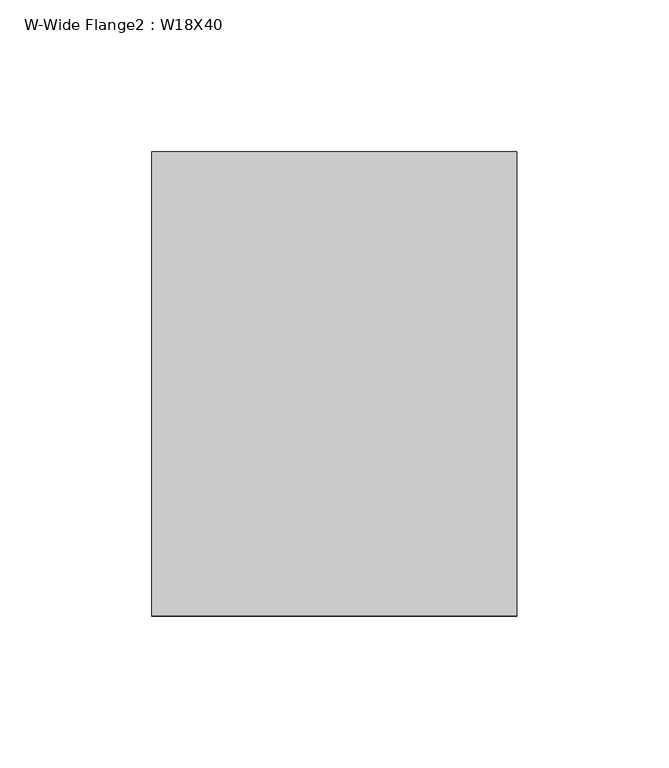
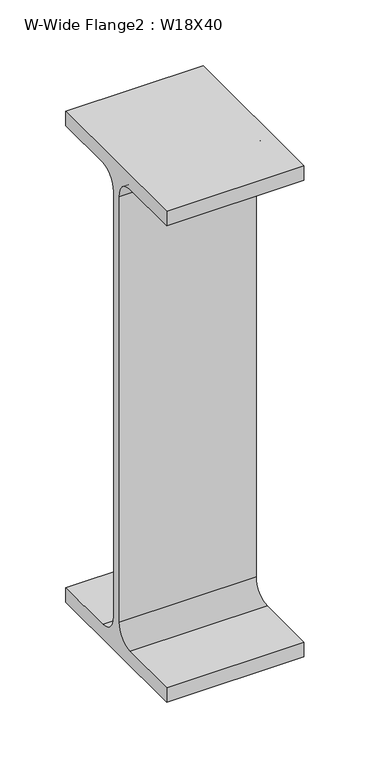
"""IFC4 building model written with IfcOpenShell, lengths in millimetres: beam geometry, W-Wide Flange2 : W18X40."""

from ifc_helpers import new_model, si_unit, point, frame, frame_2d, origin, place, context, project, spatial, polyline, circle_curve, trimmed, segment, composite_curve, outline, extrude, source, transform, mapped, element, save


def w_wide_flange2_w18x40_cc527176(model_context):
    return source(origin(), model_context, "Body", "SweptSolid", [
        extrude(outline(composite_curve([segment(polyline([(76.454, -213.995), (76.454, -227.33), (-76.454, -227.33), (-76.454, -213.995), (-20.828, -213.995)]), True, "CONTINUOUS"), segment(trimmed(circle_curve(frame_2d((-20.828, -197.1675)), 16.8275), [point((-20.828, -213.995))], [point((-4.0005, -197.1675))], True, "CARTESIAN"), True, "CONTINUOUS"), segment(polyline([(-4.0005, -197.1675), (-4.0005, 197.1675)]), True, "CONTINUOUS"), segment(trimmed(circle_curve(frame_2d((-20.828, 197.1675)), 16.8275), [point((-4.0005, 197.1675))], [point((-20.828, 213.995))], True, "CARTESIAN"), True, "CONTINUOUS"), segment(polyline([(-20.828, 213.995), (-76.454, 213.995), (-76.454, 227.33), (76.454, 227.33), (76.454, 213.995), (20.828, 213.995)]), True, "CONTINUOUS"), segment(trimmed(circle_curve(frame_2d((20.828, 197.1675)), 16.8275), [point((20.828, 213.995))], [point((4.0005, 197.1675))], True, "CARTESIAN"), True, "CONTINUOUS"), segment(polyline([(4.0005, 197.1675), (4.0005, -197.1675)]), True, "CONTINUOUS"), segment(trimmed(circle_curve(frame_2d((20.828, -197.1675)), 16.8275), [point((4.0005, -197.1675))], [point((20.828, -213.995))], True, "CARTESIAN"), True, "CONTINUOUS"), segment(polyline([(20.828, -213.995), (76.454, -213.995)]), True, "CONTINUOUS")], self_intersect=False)), frame((-91.28125, 0.0, 0.0), z_axis=(1.0, 0.0, 0.0), x_axis=(0.0, 1.0, 0.0)), (0.0, 0.0, 1.0), 120.253125),
    ])


if __name__ == "__main__":
    model = new_model("IFC4")
    model_context = context("Model", 3, world=origin())
    ifc_project = project(units=[si_unit("LENGTHUNIT", "METRE", prefix="MILLI")], contexts=[model_context])
    site = spatial("IfcSite", under=ifc_project)
    building = spatial("IfcBuilding", under=site)
    placement = place(None, origin())
    w_wide_flange2_w18x40_shape = w_wide_flange2_w18x40_cc527176(model_context)
    element("IfcBeam", 1, ObjectType="W-Wide Flange2 : W18X40", at=placement, inside=building, context=model_context, shape_type="MappedRepresentation", body=[
        mapped(w_wide_flange2_w18x40_shape, transform((0.0, 0.0, 0.0), x_axis=(1.0, 0.0, 0.0), y_axis=(0.0, 1.0, 0.0), z_axis=(0.0, 0.0, 1.0))),
    ])
    save(model, "model.ifc")

# Revit data of these elements
# Type "W-Wide Flange2 : W18X40"
#   Assembly Code = "B10"
#   W = 40
#   Length [instance default] = 5' - 0"
#   bf = 0' - 6.02"
#   d = 1' - 5.9"
#   k = 0' - 1 3/16"
#   k2 = 0' - 0.6625"
#   tf = 0' - 0.525"
#   tw = 0' - 0.315"
#   A = 0.0819444 SF
#   Structural Material [instance default] = Steel ASTM A992
# Element 1 (IfcBeam, "W-Wide Flange2 : W18X40")
#   Materials on its faces: "Steel ASTM A992"
# Materials
#   "Steel ASTM A992": class "Metal", colour RGB 199 199 199, transparency 0, Description = "Structural steel 50ksi", Cost = 0
